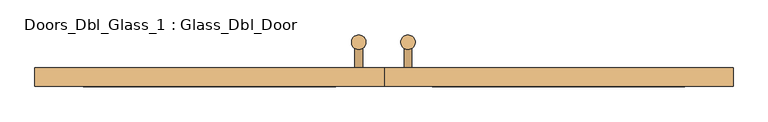
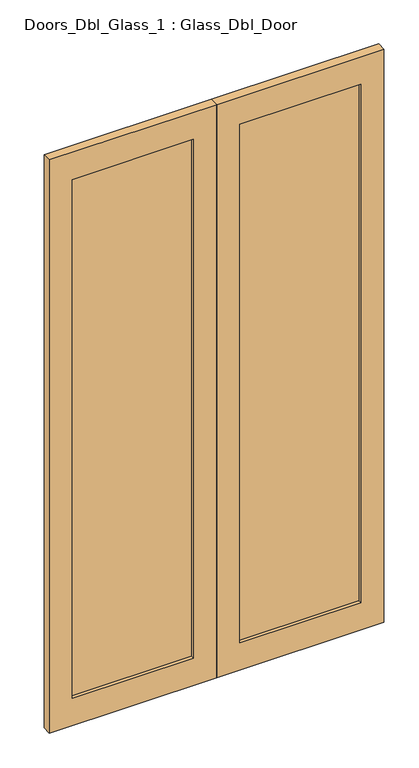
"""IFC4 building model written with IfcOpenShell, lengths in millimetres: door geometry, Doors_Dbl_Glass_1 : Glass_Dbl_Door."""

from ifc_helpers import new_model, si_unit, point, frame, frame_2d, origin, place, context, project, spatial, polyline, circle_curve, trimmed, segment, composite_curve, outline, extrude, source, transform, mapped, element, save


def doors_dbl_glass_1_glass_dbl_door_2c6c785a(model_context):
    return source(origin(), model_context, "Body", "SweptSolid", [
        extrude(outline(composite_curve([segment(trimmed(circle_curve(frame_2d((49.6069979, 116.0715804)), 15.0), [point((49.6069979, 101.0715804))], [point((49.6069979, 131.0715804))], False, "CARTESIAN"), True, "CONTINUOUS"), segment(trimmed(circle_curve(frame_2d((49.6069979, 116.0715804)), 15.0), [point((49.6069979, 131.0715804))], [point((49.6069979, 101.0715804))], False, "CARTESIAN"), True, "CONTINUOUS")], self_intersect=False)), frame((0.0, 0.0, 650.0), z_axis=(0.0, 0.0, 1.0), x_axis=(1.0, 0.0, 0.0)), (0.0, 0.0, 1.0), 900.0),
        extrude(outline(composite_curve([segment(trimmed(circle_curve(frame_2d((-52.537897, 116.0715804)), 15.0), [point((-52.537897, 101.0715804))], [point((-52.537897, 131.0715804))], False, "CARTESIAN"), True, "CONTINUOUS"), segment(trimmed(circle_curve(frame_2d((-52.537897, 116.0715804)), 15.0), [point((-52.537897, 131.0715804))], [point((-52.537897, 101.0715804))], False, "CARTESIAN"), True, "CONTINUOUS")], self_intersect=False)), frame((0.0, 0.0, 650.0), z_axis=(0.0, 0.0, 1.0), x_axis=(1.0, 0.0, 0.0)), (0.0, 0.0, 1.0), 900.0),
        extrude(outline(composite_curve([segment(trimmed(circle_curve(frame_2d((750.0, 49.6069979)), 8.0), [point((750.0, 57.6069979))], [point((750.0, 41.6069979))], False, "CARTESIAN"), True, "CONTINUOUS"), segment(trimmed(circle_curve(frame_2d((750.0, 49.6069979)), 8.0), [point((750.0, 41.6069979))], [point((750.0, 57.6069979))], False, "CARTESIAN"), True, "CONTINUOUS")], self_intersect=False)), frame((0.0, 62.5788556, 0.0), z_axis=(0.0, 1.0, 0.0), x_axis=(0.0, 0.0, 1.0)), (0.0, 0.0, 1.0), 53.4927248),
        extrude(outline(composite_curve([segment(trimmed(circle_curve(frame_2d((750.0, -52.537897)), 8.0), [point((750.0, -44.537897))], [point((750.0, -60.537897))], False, "CARTESIAN"), True, "CONTINUOUS"), segment(trimmed(circle_curve(frame_2d((750.0, -52.537897)), 8.0), [point((750.0, -60.537897))], [point((750.0, -44.537897))], False, "CARTESIAN"), True, "CONTINUOUS")], self_intersect=False)), frame((0.0, 62.5788556, 0.0), z_axis=(0.0, 1.0, 0.0), x_axis=(0.0, 0.0, 1.0)), (0.0, 0.0, 1.0), 53.4927248),
        extrude(outline(composite_curve([segment(trimmed(circle_curve(frame_2d((1450.0, 49.6069979)), 8.0), [point((1450.0, 57.6069979))], [point((1450.0, 41.6069979))], False, "CARTESIAN"), True, "CONTINUOUS"), segment(trimmed(circle_curve(frame_2d((1450.0, 49.6069979)), 8.0), [point((1450.0, 41.6069979))], [point((1450.0, 57.6069979))], False, "CARTESIAN"), True, "CONTINUOUS")], self_intersect=False)), frame((0.0, 62.5788556, 0.0), z_axis=(0.0, 1.0, 0.0), x_axis=(0.0, 0.0, 1.0)), (0.0, 0.0, 1.0), 53.4927248),
        extrude(outline(composite_curve([segment(trimmed(circle_curve(frame_2d((1450.0, -52.537897)), 8.0), [point((1450.0, -44.537897))], [point((1450.0, -60.537897))], False, "CARTESIAN"), True, "CONTINUOUS"), segment(trimmed(circle_curve(frame_2d((1450.0, -52.537897)), 8.0), [point((1450.0, -60.537897))], [point((1450.0, -44.537897))], False, "CARTESIAN"), True, "CONTINUOUS")], self_intersect=False)), frame((0.0, 62.5788556, 0.0), z_axis=(0.0, 1.0, 0.0), x_axis=(0.0, 0.0, 1.0)), (0.0, 0.0, 1.0), 53.4927248),
        extrude(outline(polyline([(2625.0, -724.9999999), (0.0, -724.9999999), (0.0, 0.0), (2625.0, 0.0), (2625.0, -724.9999999)]), holes=[polyline([(2500.0, -624.9999999), (2500.0, -100.0), (125.0, -100.0), (125.0, -624.9999999), (2500.0, -624.9999999)])]), frame((0.0, 24.035259, 0.0), z_axis=(0.0, 1.0, 0.0), x_axis=(0.0, 0.0, 1.0)), (0.0, 0.0, 1.0), 38.5435966),
        extrude(outline(polyline([(2625.0, 0.0), (0.0, 0.0), (0.0, 724.9999999), (2625.0, 724.9999999), (2625.0, 0.0)]), holes=[polyline([(2500.0, 100.0), (2500.0, 624.9999999), (125.0, 624.9999999), (125.0, 100.0), (2500.0, 100.0)])]), frame((0.0, 24.035259, 0.0), z_axis=(0.0, 1.0, 0.0), x_axis=(0.0, 0.0, 1.0)), (0.0, 0.0, 1.0), 38.5435966),
        extrude(outline(polyline([(-100.0, 38.0), (-624.9999999, 38.0), (-624.9999999, 50.0), (-100.0, 50.0), (-100.0, 38.0)])), frame((0.0, 0.0, 125.0), z_axis=(0.0, 0.0, 1.0), x_axis=(1.0, 0.0, 0.0)), (0.0, 0.0, 1.0), 2375.0),
        extrude(outline(polyline([(624.9999999, 38.0), (100.0, 38.0), (100.0, 50.0), (624.9999999, 50.0), (624.9999999, 38.0)])), frame((0.0, 0.0, 125.0), z_axis=(0.0, 0.0, 1.0), x_axis=(1.0, 0.0, 0.0)), (0.0, 0.0, 1.0), 2375.0),
    ])


if __name__ == "__main__":
    model = new_model("IFC4")
    model_context = context("Model", 3, world=origin())
    ifc_project = project(units=[si_unit("LENGTHUNIT", "METRE", prefix="MILLI")], contexts=[model_context])
    site = spatial("IfcSite", under=ifc_project)
    building = spatial("IfcBuilding", under=site)
    placement = place(None, origin())
    doors_dbl_glass_1_glass_dbl_door_shape = doors_dbl_glass_1_glass_dbl_door_2c6c785a(model_context)
    element("IfcDoor", 1, ObjectType="Doors_Dbl_Glass_1 : Glass_Dbl_Door", at=placement, inside=building, context=model_context, shape_type="MappedRepresentation", body=[
        mapped(doors_dbl_glass_1_glass_dbl_door_shape, transform((0.0, 0.0, 0.0), x_axis=(1.0, 0.0, 0.0), y_axis=(0.0, 1.0, 0.0), z_axis=(0.0, 0.0, 1.0))),
    ])
    save(model, "model.ifc")

# Revit data of these elements
# Type "Doors_Dbl_Glass_1 : Glass_Dbl_Door"
#   Type Mark = "48"
#   Construction Type Id = "GSP4R"
#   Analytic Construction = "1/8 in Pilkington single glazing"
#   Visual Light Transmittance = 0.9
#   Stile Shutting = 100 mm
#   Stile Hanging = 100 mm
#   Stile - Top Rail = 125 mm
#   Stile - Bottom Rail = 125 mm
#   Solar Heat Gain Coefficient = 0.78
#   Offset = 50 mm
#   Heat Transfer Coefficient (U) = 3.6886 W/(m²·K)
#   Glass Thickness = 12 mm
#   Define Thermal Properties by = 1
#   Material Ironmongery = Metal - Aluminum
#   Material Door = Metal - Aluminum
#   Material Glass = Glass
#   Function = (empty or 0)
# Element 1 (IfcDoor, "Doors_Dbl_Glass_1 : Glass_Dbl_Door")
#   Materials on its faces: "Metal - Aluminum", "Glass"
# Materials
#   "Metal - Aluminum": class "Metal", colour RGB 247 247 247, transparency 0
#   "Glass": class "Glass", colour RGB 0 128 192, transparency 0.9, Description = "Soda Lime Glass", Cost = 0
